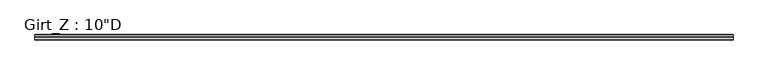
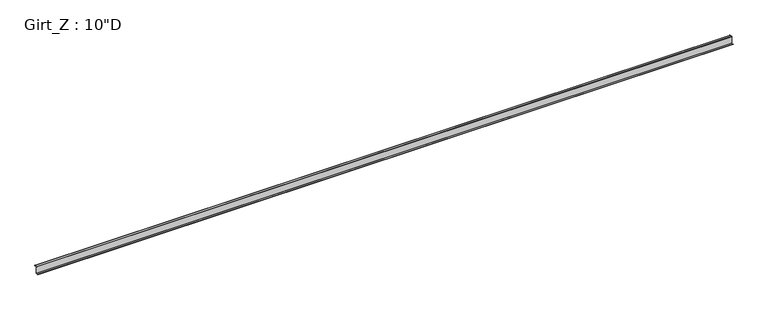
"""IFC4 building model written with IfcOpenShell, lengths in millimetres: beam geometry."""

from ifc_helpers import new_model, si_unit, point, frame, frame_2d, origin, place, context, project, spatial, polyline, circle_curve, trimmed, segment, composite_curve, outline, extrude, source, transform, mapped, element, save


def beam_302408e8(model_context):
    return source(origin(), model_context, "Body", "SweptSolid", [
        extrude(outline(composite_curve([segment(polyline([(77.9859375, 127.0), (90.2310415, 112.4068534), (88.1028742, 110.621109), (76.6904765, 124.221875), (3.3005807, 124.221875)]), True, "CONTINUOUS"), segment(trimmed(circle_curve(frame_2d((3.3741066, 122.2381931)), 1.9850441), [point((3.3005807, 124.221875))], [point((1.3890625, 122.2381931))], True, "CARTESIAN"), True, "CONTINUOUS"), segment(polyline([(1.3890625, 122.2381931), (1.3890625, -127.0), (-84.3359375, -127.0), (-96.5810415, -112.4068534), (-94.4528742, -110.621109), (-83.0404765, -124.221875), (-3.2694106, -124.221875)]), True, "CONTINUOUS"), segment(trimmed(circle_curve(frame_2d((-3.3748024, -122.2389339)), 1.9857399), [point((-3.2694106, -124.221875))], [point((-1.3890625, -122.2389339))], True, "CARTESIAN"), True, "CONTINUOUS"), segment(polyline([(-1.3890625, -122.2389339), (-1.3890625, 122.2375)]), True, "CONTINUOUS"), segment(trimmed(circle_curve(frame_2d((3.3734375, 122.2375)), 4.7625), [point((-1.3890625, 122.2375))], [point((3.3734375, 127.0))], False, "CARTESIAN"), True, "CONTINUOUS"), segment(polyline([(3.3734375, 127.0), (77.9859375, 127.0)]), True, "CONTINUOUS")], self_intersect=False)), frame((-12455.525, 0.0, 0.0), z_axis=(1.0, 0.0, 0.0), x_axis=(0.0, 1.0, 0.0)), (0.0, 0.0, 1.0), 24739.6),
    ])


if __name__ == "__main__":
    model = new_model("IFC4")
    model_context = context("Model", 3, world=origin())
    ifc_project = project(units=[si_unit("LENGTHUNIT", "METRE", prefix="MILLI")], contexts=[model_context])
    site = spatial("IfcSite", under=ifc_project)
    building = spatial("IfcBuilding", under=site)
    placement = place(None, origin())
    beam_shape = beam_302408e8(model_context)
    element("IfcBeam", 1, ObjectType="Girt_Z : 10\"D", at=placement, inside=building, context=model_context, shape_type="MappedRepresentation", body=[
        mapped(beam_shape, transform((0.0, 0.0, 0.0), x_axis=(1.0, 0.0, 0.0), y_axis=(0.0, 1.0, 0.0), z_axis=(0.0, 0.0, 1.0))),
    ])
    save(model, "model.ifc")

# Revit data of these elements
# Type "Girt_Z : 10\"D"
#   half leg = 0' - 1 11/16"
#   Web_Thickness = 0' - 0 7/64"
#   Length [instance default] = 10' - 0"
#   Leg_2 = 0' - 3 3/8"
#   Leg_1 = 0' - 3 1/8"
#   Height = 0' - 10"
#   Structural Material [instance default] = none
# Element 1 (IfcBeam, "Girt_Z : 10\"D")
#   Structural Material = STRUCTURAL STEEL - SEE STRUCT. DWGS
#   Materials on its faces: "STRUCTURAL STEEL - SEE STRUCT. DWGS"
# Materials
#   "STRUCTURAL STEEL - SEE STRUCT. DWGS": class "Metal", colour RGB 137 146 153, transparency 0, Description = "Steel, mill finish", Cost = 0
